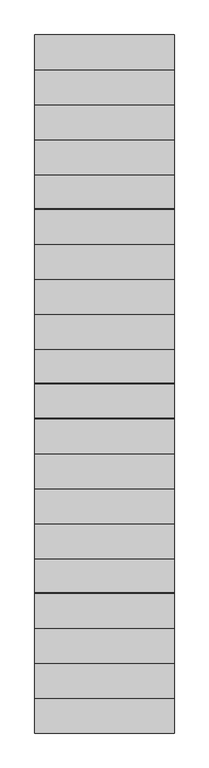
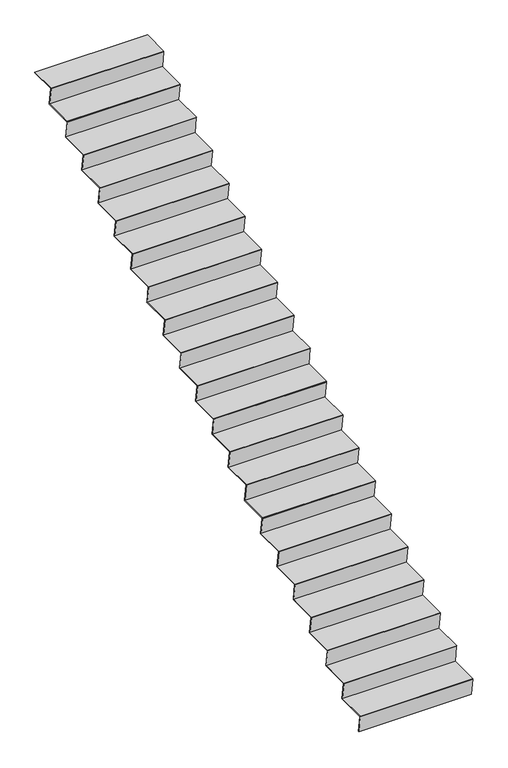
"""IFC4 building model written with IfcOpenShell, lengths in millimetres: stair flight geometry."""

from ifc_helpers import new_model, si_unit, frame, origin, place, context, project, spatial, polyline, outline, extrude, source, transform, mapped, element, save


def stair_flight_cf0df241(model_context):
    return source(origin(), model_context, "Body", "SweptSolid", [
        extrude(outline(polyline([(-16698.7691378, 695.6521739), (-16392.7074626, 695.6521739), (-16391.8449626, 689.6521739), (-16697.9066378, 689.6521739), (-16698.7691378, 695.6521739)])), frame((15747.5726879, 0.0, 0.0), z_axis=(1.0, 0.0, 0.0), x_axis=(0.0, 1.0, 0.0)), (0.0, 0.0, 1.0), 1100.0),
        extrude(outline(polyline([(-16697.9066378, 689.6521739), (-16691.8449626, 689.6521739), (-16667.7074626, 521.7391304), (-16673.7691378, 521.7391304), (-16697.9066378, 689.6521739)])), frame((15747.5726879, 0.0, 0.0), z_axis=(1.0, 0.0, 0.0), x_axis=(0.0, 1.0, 0.0)), (0.0, 0.0, 1.0), 1100.0),
        extrude(outline(polyline([(-16422.9066378, 863.5652174), (-16416.8449626, 863.5652174), (-16392.7074626, 695.6521739), (-16398.7691378, 695.6521739), (-16422.9066378, 863.5652174)])), frame((15747.5726879, 0.0, 0.0), z_axis=(1.0, 0.0, 0.0), x_axis=(0.0, 1.0, 0.0)), (0.0, 0.0, 1.0), 1100.0),
        extrude(outline(polyline([(-16423.7691378, 869.5652174), (-16117.7074626, 869.5652174), (-16116.8449626, 863.5652174), (-16422.9066378, 863.5652174), (-16423.7691378, 869.5652174)])), frame((15747.5726879, 0.0, 0.0), z_axis=(1.0, 0.0, 0.0), x_axis=(0.0, 1.0, 0.0)), (0.0, 0.0, 1.0), 1100.0),
        extrude(outline(polyline([(-16147.9066378, 1037.4782609), (-16141.8449626, 1037.4782609), (-16117.7074626, 869.5652174), (-16123.7691378, 869.5652174), (-16147.9066378, 1037.4782609)])), frame((15747.5726879, 0.0, 0.0), z_axis=(1.0, 0.0, 0.0), x_axis=(0.0, 1.0, 0.0)), (0.0, 0.0, 1.0), 1100.0),
        extrude(outline(polyline([(-16148.7691378, 1043.4782609), (-15842.7074626, 1043.4782609), (-15841.8449626, 1037.4782609), (-16147.9066378, 1037.4782609), (-16148.7691378, 1043.4782609)])), frame((15747.5726879, 0.0, 0.0), z_axis=(1.0, 0.0, 0.0), x_axis=(0.0, 1.0, 0.0)), (0.0, 0.0, 1.0), 1100.0),
        extrude(outline(polyline([(-15872.9066378, 1211.3913043), (-15866.8449626, 1211.3913043), (-15842.7074626, 1043.4782609), (-15848.7691378, 1043.4782609), (-15872.9066378, 1211.3913043)])), frame((15747.5726879, 0.0, 0.0), z_axis=(1.0, 0.0, 0.0), x_axis=(0.0, 1.0, 0.0)), (0.0, 0.0, 1.0), 1100.0),
        extrude(outline(polyline([(-15873.7691378, 1217.3913043), (-15567.7074626, 1217.3913043), (-15566.8449626, 1211.3913043), (-15872.9066378, 1211.3913043), (-15873.7691378, 1217.3913043)])), frame((15747.5726879, 0.0, 0.0), z_axis=(1.0, 0.0, 0.0), x_axis=(0.0, 1.0, 0.0)), (0.0, 0.0, 1.0), 1100.0),
        extrude(outline(polyline([(-15597.9066378, 1385.3043478), (-15591.8449626, 1385.3043478), (-15567.7074626, 1217.3913043), (-15573.7691378, 1217.3913043), (-15597.9066378, 1385.3043478)])), frame((15747.5726879, 0.0, 0.0), z_axis=(1.0, 0.0, 0.0), x_axis=(0.0, 1.0, 0.0)), (0.0, 0.0, 1.0), 1100.0),
        extrude(outline(polyline([(-15598.7691378, 1391.3043478), (-15292.7074626, 1391.3043478), (-15291.8449626, 1385.3043478), (-15597.9066378, 1385.3043478), (-15598.7691378, 1391.3043478)])), frame((15747.5726879, 0.0, 0.0), z_axis=(1.0, 0.0, 0.0), x_axis=(0.0, 1.0, 0.0)), (0.0, 0.0, 1.0), 1100.0),
        extrude(outline(polyline([(-15322.9066378, 1559.2173913), (-15316.8449626, 1559.2173913), (-15292.7074626, 1391.3043478), (-15298.7691378, 1391.3043478), (-15322.9066378, 1559.2173913)])), frame((15747.5726879, 0.0, 0.0), z_axis=(1.0, 0.0, 0.0), x_axis=(0.0, 1.0, 0.0)), (0.0, 0.0, 1.0), 1100.0),
        extrude(outline(polyline([(-15323.7691378, 1565.2173913), (-15017.7074626, 1565.2173913), (-15016.8449626, 1559.2173913), (-15322.9066378, 1559.2173913), (-15323.7691378, 1565.2173913)])), frame((15747.5726879, 0.0, 0.0), z_axis=(1.0, 0.0, 0.0), x_axis=(0.0, 1.0, 0.0)), (0.0, 0.0, 1.0), 1100.0),
        extrude(outline(polyline([(-15047.9066378, 1733.1304348), (-15041.8449626, 1733.1304348), (-15017.7074626, 1565.2173913), (-15023.7691378, 1565.2173913), (-15047.9066378, 1733.1304348)])), frame((15747.5726879, 0.0, 0.0), z_axis=(1.0, 0.0, 0.0), x_axis=(0.0, 1.0, 0.0)), (0.0, 0.0, 1.0), 1100.0),
        extrude(outline(polyline([(-15048.7691378, 1739.1304348), (-14742.7074626, 1739.1304348), (-14741.8449626, 1733.1304348), (-15047.9066378, 1733.1304348), (-15048.7691378, 1739.1304348)])), frame((15747.5726879, 0.0, 0.0), z_axis=(1.0, 0.0, 0.0), x_axis=(0.0, 1.0, 0.0)), (0.0, 0.0, 1.0), 1100.0),
        extrude(outline(polyline([(-14772.9066378, 1907.0434783), (-14766.8449626, 1907.0434783), (-14742.7074626, 1739.1304348), (-14748.7691378, 1739.1304348), (-14772.9066378, 1907.0434783)])), frame((15747.5726879, 0.0, 0.0), z_axis=(1.0, 0.0, 0.0), x_axis=(0.0, 1.0, 0.0)), (0.0, 0.0, 1.0), 1100.0),
        extrude(outline(polyline([(-14773.7691378, 1913.0434783), (-14467.7074626, 1913.0434783), (-14466.8449626, 1907.0434783), (-14772.9066378, 1907.0434783), (-14773.7691378, 1913.0434783)])), frame((15747.5726879, 0.0, 0.0), z_axis=(1.0, 0.0, 0.0), x_axis=(0.0, 1.0, 0.0)), (0.0, 0.0, 1.0), 1100.0),
        extrude(outline(polyline([(-14497.9066378, 2080.9565217), (-14491.8449626, 2080.9565217), (-14467.7074626, 1913.0434783), (-14473.7691378, 1913.0434783), (-14497.9066378, 2080.9565217)])), frame((15747.5726879, 0.0, 0.0), z_axis=(1.0, 0.0, 0.0), x_axis=(0.0, 1.0, 0.0)), (0.0, 0.0, 1.0), 1100.0),
        extrude(outline(polyline([(-14498.7691378, 2086.9565217), (-14192.7074626, 2086.9565217), (-14191.8449626, 2080.9565217), (-14497.9066378, 2080.9565217), (-14498.7691378, 2086.9565217)])), frame((15747.5726879, 0.0, 0.0), z_axis=(1.0, 0.0, 0.0), x_axis=(0.0, 1.0, 0.0)), (0.0, 0.0, 1.0), 1100.0),
        extrude(outline(polyline([(-14222.9066378, 2254.8695652), (-14216.8449626, 2254.8695652), (-14192.7074626, 2086.9565217), (-14198.7691378, 2086.9565217), (-14222.9066378, 2254.8695652)])), frame((15747.5726879, 0.0, 0.0), z_axis=(1.0, 0.0, 0.0), x_axis=(0.0, 1.0, 0.0)), (0.0, 0.0, 1.0), 1100.0),
        extrude(outline(polyline([(-14223.7691378, 2260.8695652), (-13917.7074626, 2260.8695652), (-13916.8449626, 2254.8695652), (-14222.9066378, 2254.8695652), (-14223.7691378, 2260.8695652)])), frame((15747.5726879, 0.0, 0.0), z_axis=(1.0, 0.0, 0.0), x_axis=(0.0, 1.0, 0.0)), (0.0, 0.0, 1.0), 1100.0),
        extrude(outline(polyline([(-13947.9066378, 2428.7826087), (-13941.8449626, 2428.7826087), (-13917.7074626, 2260.8695652), (-13923.7691378, 2260.8695652), (-13947.9066378, 2428.7826087)])), frame((15747.5726879, 0.0, 0.0), z_axis=(1.0, 0.0, 0.0), x_axis=(0.0, 1.0, 0.0)), (0.0, 0.0, 1.0), 1100.0),
        extrude(outline(polyline([(-13948.7691378, 2434.7826087), (-13642.7074626, 2434.7826087), (-13641.8449626, 2428.7826087), (-13947.9066378, 2428.7826087), (-13948.7691378, 2434.7826087)])), frame((15747.5726879, 0.0, 0.0), z_axis=(1.0, 0.0, 0.0), x_axis=(0.0, 1.0, 0.0)), (0.0, 0.0, 1.0), 1100.0),
        extrude(outline(polyline([(-13672.9066378, 2602.6956522), (-13666.8449626, 2602.6956522), (-13642.7074626, 2434.7826087), (-13648.7691378, 2434.7826087), (-13672.9066378, 2602.6956522)])), frame((15747.5726879, 0.0, 0.0), z_axis=(1.0, 0.0, 0.0), x_axis=(0.0, 1.0, 0.0)), (0.0, 0.0, 1.0), 1100.0),
        extrude(outline(polyline([(-13673.7691378, 2608.6956522), (-13367.7074626, 2608.6956522), (-13366.8449626, 2602.6956522), (-13672.9066378, 2602.6956522), (-13673.7691378, 2608.6956522)])), frame((15747.5726879, 0.0, 0.0), z_axis=(1.0, 0.0, 0.0), x_axis=(0.0, 1.0, 0.0)), (0.0, 0.0, 1.0), 1100.0),
        extrude(outline(polyline([(-13397.9066378, 2776.6086957), (-13391.8449626, 2776.6086957), (-13367.7074626, 2608.6956522), (-13373.7691378, 2608.6956522), (-13397.9066378, 2776.6086957)])), frame((15747.5726879, 0.0, 0.0), z_axis=(1.0, 0.0, 0.0), x_axis=(0.0, 1.0, 0.0)), (0.0, 0.0, 1.0), 1100.0),
        extrude(outline(polyline([(-13398.7691378, 2782.6086957), (-13092.7074626, 2782.6086957), (-13091.8449626, 2776.6086957), (-13397.9066378, 2776.6086957), (-13398.7691378, 2782.6086957)])), frame((15747.5726879, 0.0, 0.0), z_axis=(1.0, 0.0, 0.0), x_axis=(0.0, 1.0, 0.0)), (0.0, 0.0, 1.0), 1100.0),
        extrude(outline(polyline([(-13122.9066378, 2950.5217391), (-13116.8449626, 2950.5217391), (-13092.7074626, 2782.6086957), (-13098.7691378, 2782.6086957), (-13122.9066378, 2950.5217391)])), frame((15747.5726879, 0.0, 0.0), z_axis=(1.0, 0.0, 0.0), x_axis=(0.0, 1.0, 0.0)), (0.0, 0.0, 1.0), 1100.0),
        extrude(outline(polyline([(-13123.7691378, 2956.5217391), (-12817.7074626, 2956.5217391), (-12816.8449626, 2950.5217391), (-13122.9066378, 2950.5217391), (-13123.7691378, 2956.5217391)])), frame((15747.5726879, 0.0, 0.0), z_axis=(1.0, 0.0, 0.0), x_axis=(0.0, 1.0, 0.0)), (0.0, 0.0, 1.0), 1100.0),
        extrude(outline(polyline([(-12847.9066378, 3124.4347826), (-12841.8449626, 3124.4347826), (-12817.7074626, 2956.5217391), (-12823.7691378, 2956.5217391), (-12847.9066378, 3124.4347826)])), frame((15747.5726879, 0.0, 0.0), z_axis=(1.0, 0.0, 0.0), x_axis=(0.0, 1.0, 0.0)), (0.0, 0.0, 1.0), 1100.0),
        extrude(outline(polyline([(-12848.7691378, 3130.4347826), (-12542.7074626, 3130.4347826), (-12541.8449626, 3124.4347826), (-12847.9066378, 3124.4347826), (-12848.7691378, 3130.4347826)])), frame((15747.5726879, 0.0, 0.0), z_axis=(1.0, 0.0, 0.0), x_axis=(0.0, 1.0, 0.0)), (0.0, 0.0, 1.0), 1100.0),
        extrude(outline(polyline([(-12572.9066378, 3298.3478261), (-12566.8449626, 3298.3478261), (-12542.7074626, 3130.4347826), (-12548.7691378, 3130.4347826), (-12572.9066378, 3298.3478261)])), frame((15747.5726879, 0.0, 0.0), z_axis=(1.0, 0.0, 0.0), x_axis=(0.0, 1.0, 0.0)), (0.0, 0.0, 1.0), 1100.0),
        extrude(outline(polyline([(-12573.7691378, 3304.3478261), (-12267.7074626, 3304.3478261), (-12266.8449626, 3298.3478261), (-12572.9066378, 3298.3478261), (-12573.7691378, 3304.3478261)])), frame((15747.5726879, 0.0, 0.0), z_axis=(1.0, 0.0, 0.0), x_axis=(0.0, 1.0, 0.0)), (0.0, 0.0, 1.0), 1100.0),
        extrude(outline(polyline([(-12297.9066378, 3472.2608696), (-12291.8449626, 3472.2608696), (-12267.7074626, 3304.3478261), (-12273.7691378, 3304.3478261), (-12297.9066378, 3472.2608696)])), frame((15747.5726879, 0.0, 0.0), z_axis=(1.0, 0.0, 0.0), x_axis=(0.0, 1.0, 0.0)), (0.0, 0.0, 1.0), 1100.0),
        extrude(outline(polyline([(-12298.7691378, 3478.2608696), (-11992.7074626, 3478.2608696), (-11991.8449626, 3472.2608696), (-12297.9066378, 3472.2608696), (-12298.7691378, 3478.2608696)])), frame((15747.5726879, 0.0, 0.0), z_axis=(1.0, 0.0, 0.0), x_axis=(0.0, 1.0, 0.0)), (0.0, 0.0, 1.0), 1100.0),
        extrude(outline(polyline([(-12022.9066378, 3646.173913), (-12016.8449626, 3646.173913), (-11992.7074626, 3478.2608696), (-11998.7691378, 3478.2608696), (-12022.9066378, 3646.173913)])), frame((15747.5726879, 0.0, 0.0), z_axis=(1.0, 0.0, 0.0), x_axis=(0.0, 1.0, 0.0)), (0.0, 0.0, 1.0), 1100.0),
        extrude(outline(polyline([(-12023.7691378, 3652.173913), (-11717.7074626, 3652.173913), (-11716.8449626, 3646.173913), (-12022.9066378, 3646.173913), (-12023.7691378, 3652.173913)])), frame((15747.5726879, 0.0, 0.0), z_axis=(1.0, 0.0, 0.0), x_axis=(0.0, 1.0, 0.0)), (0.0, 0.0, 1.0), 1100.0),
        extrude(outline(polyline([(-11747.9066378, 3820.0869565), (-11741.8449626, 3820.0869565), (-11717.7074626, 3652.173913), (-11723.7691378, 3652.173913), (-11747.9066378, 3820.0869565)])), frame((15747.5726879, 0.0, 0.0), z_axis=(1.0, 0.0, 0.0), x_axis=(0.0, 1.0, 0.0)), (0.0, 0.0, 1.0), 1100.0),
        extrude(outline(polyline([(-11748.7691378, 3826.0869565), (-11442.7074626, 3826.0869565), (-11441.8449626, 3820.0869565), (-11747.9066378, 3820.0869565), (-11748.7691378, 3826.0869565)])), frame((15747.5726879, 0.0, 0.0), z_axis=(1.0, 0.0, 0.0), x_axis=(0.0, 1.0, 0.0)), (0.0, 0.0, 1.0), 1100.0),
        extrude(outline(polyline([(-11472.9066378, 3994.0), (-11466.8449626, 3994.0), (-11442.7074626, 3826.0869565), (-11448.7691378, 3826.0869565), (-11472.9066378, 3994.0)])), frame((15747.5726879, 0.0, 0.0), z_axis=(1.0, 0.0, 0.0), x_axis=(0.0, 1.0, 0.0)), (0.0, 0.0, 1.0), 1100.0),
        extrude(outline(polyline([(-11473.7691378, 4000.0), (-11198.7691378, 4000.0), (-11198.7691378, 3994.0), (-11472.9066378, 3994.0), (-11473.7691378, 4000.0)])), frame((15747.5726879, 0.0, 0.0), z_axis=(1.0, 0.0, 0.0), x_axis=(0.0, 1.0, 0.0)), (0.0, 0.0, 1.0), 1100.0),
    ])


if __name__ == "__main__":
    model = new_model("IFC4")
    model_context = context("Model", 3, world=origin())
    ifc_project = project(units=[si_unit("LENGTHUNIT", "METRE", prefix="MILLI")], contexts=[model_context])
    site = spatial("IfcSite", under=ifc_project)
    building = spatial("IfcBuilding", under=site)
    placement = place(None, origin())
    stair_flight_shape = stair_flight_cf0df241(model_context)
    element("IfcStairFlight", 1, at=placement, inside=building, context=model_context, shape_type="MappedRepresentation", body=[
        mapped(stair_flight_shape, transform((0.0, 0.0, 0.0), x_axis=(1.0, 0.0, 0.0), y_axis=(0.0, 1.0, 0.0), z_axis=(0.0, 0.0, 1.0))),
    ])
    save(model, "model.ifc")

# Revit data of these elements
# Element 1 (IfcStairFlight)
#   Materials on its faces: "Acero, acabado de pintura, gris oscuro"
# Materials
#   "Acero, acabado de pintura, gris oscuro": class "Metal", colour RGB 89 89 89, transparency 0, Description = "Acero, acabado de pintura, gris oscuro, brillante", Cost = 0
